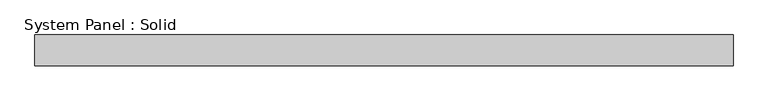
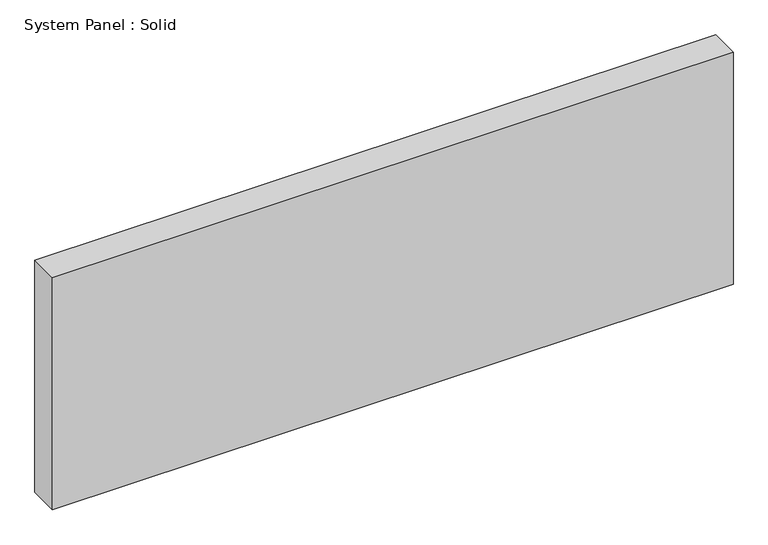
"""IFC4 building model written with IfcOpenShell, lengths in millimetres: plate geometry, System Panel : Solid."""

from ifc_helpers import new_model, si_unit, origin, origin_with_axes, place, context, project, spatial, polyline, outline, extrude, source, transform, mapped, element, save


def system_panel_solid_4932440a(model_context):
    return source(origin(), model_context, "Body", "SweptSolid", [
        extrude(outline(polyline([(713.3166666, -19.05), (-713.3166666, -19.05), (-713.3166666, 44.45), (713.3166666, 44.45), (713.3166666, -19.05)])), origin_with_axes(), (0.0, 0.0, 1.0), 514.35),
    ])


if __name__ == "__main__":
    model = new_model("IFC4")
    model_context = context("Model", 3, world=origin())
    ifc_project = project(units=[si_unit("LENGTHUNIT", "METRE", prefix="MILLI")], contexts=[model_context])
    site = spatial("IfcSite", under=ifc_project)
    building = spatial("IfcBuilding", under=site)
    placement = place(None, origin())
    system_panel_solid_shape = system_panel_solid_4932440a(model_context)
    element("IfcPlate", 1, ObjectType="System Panel : Solid", at=placement, inside=building, context=model_context, shape_type="MappedRepresentation", body=[
        mapped(system_panel_solid_shape, transform((0.0, 0.0, 0.0), x_axis=(1.0, 0.0, 0.0), y_axis=(0.0, 1.0, 0.0), z_axis=(0.0, 0.0, 1.0))),
    ])
    save(model, "model.ifc")

# Revit data of these elements
# Type "System Panel : Solid"
#   Construction Type Id = "MDOOR"
#   Analytic Construction = "Metal"
#   Visual Light Transmittance = 0
#   Solar Heat Gain Coefficient = 0
#   Heat Transfer Coefficient (U) = 0.651978 BTU/(h·ft²·°F)
#   Define Thermal Properties by = 1
# Element 1 (IfcPlate, "System Panel : Solid")
#   Materials on its faces: "Default"
# Materials
#   "Default": class "Miscellaneous", colour RGB 127 127 127, transparency 0, Cost = 0
